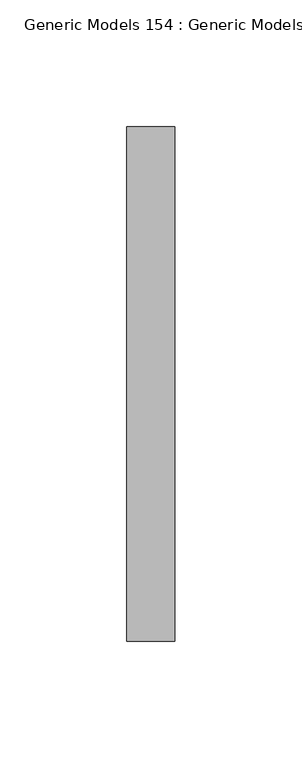
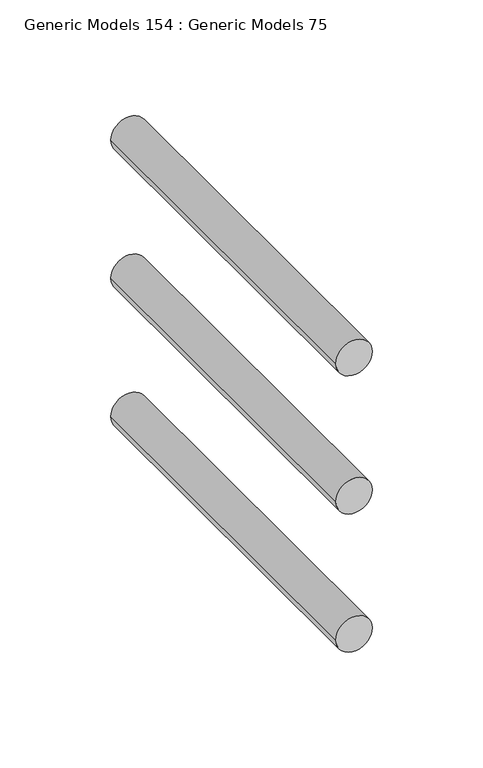
"""IFC4 building model written with IfcOpenShell, lengths in millimetres: proxy geometry, Generic Models 154 : Generic Models 75."""

from ifc_helpers import new_model, si_unit, point, frame, frame_2d, origin, place, context, project, spatial, circle_curve, trimmed, segment, composite_curve, outline, extrude, source, transform, mapped, element, save


def generic_models_154_generic_models_75_05dde245(model_context):
    return source(origin(), model_context, "Body", "SweptSolid", [
        extrude(outline(composite_curve([segment(trimmed(circle_curve(frame_2d((271689.5125, 31705.5346032)), 9.525), [point((271689.5125, 31715.0596032))], [point((271689.5125, 31696.0096032))], False, "CARTESIAN"), True, "CONTINUOUS"), segment(trimmed(circle_curve(frame_2d((271689.5125, 31705.5346032)), 9.525), [point((271689.5125, 31696.0096032))], [point((271689.5125, 31715.0596032))], False, "CARTESIAN"), True, "CONTINUOUS")], self_intersect=False)), frame((0.0, 36305.8207942, 0.0), z_axis=(0.0, 1.0, 0.0), x_axis=(0.0, 0.0, 1.0)), (0.0, 0.0, 1.0), 203.2),
        extrude(outline(composite_curve([segment(trimmed(circle_curve(frame_2d((271765.7125, 31705.5346032)), 9.525), [point((271765.7125, 31715.0596032))], [point((271765.7125, 31696.0096032))], False, "CARTESIAN"), True, "CONTINUOUS"), segment(trimmed(circle_curve(frame_2d((271765.7125, 31705.5346032)), 9.525), [point((271765.7125, 31696.0096032))], [point((271765.7125, 31715.0596032))], False, "CARTESIAN"), True, "CONTINUOUS")], self_intersect=False)), frame((0.0, 36305.8207942, 0.0), z_axis=(0.0, 1.0, 0.0), x_axis=(0.0, 0.0, 1.0)), (0.0, 0.0, 1.0), 203.2),
        extrude(outline(composite_curve([segment(trimmed(circle_curve(frame_2d((271841.9125, 31705.5346032)), 9.525), [point((271841.9125, 31715.0596032))], [point((271841.9125, 31696.0096032))], False, "CARTESIAN"), True, "CONTINUOUS"), segment(trimmed(circle_curve(frame_2d((271841.9125, 31705.5346032)), 9.525), [point((271841.9125, 31696.0096032))], [point((271841.9125, 31715.0596032))], False, "CARTESIAN"), True, "CONTINUOUS")], self_intersect=False)), frame((0.0, 36305.8207942, 0.0), z_axis=(0.0, 1.0, 0.0), x_axis=(0.0, 0.0, 1.0)), (0.0, 0.0, 1.0), 203.2),
    ])


if __name__ == "__main__":
    model = new_model("IFC4")
    model_context = context("Model", 3, world=origin())
    ifc_project = project(units=[si_unit("LENGTHUNIT", "METRE", prefix="MILLI")], contexts=[model_context])
    site = spatial("IfcSite", under=ifc_project)
    building = spatial("IfcBuilding", under=site)
    placement = place(None, origin())
    generic_models_154_generic_models_75_shape = generic_models_154_generic_models_75_05dde245(model_context)
    element("IfcBuildingElementProxy", 1, Name="Generic Models 154 : Generic Models 75", ObjectType="Generic Models 154 : Generic Models 75", at=placement, inside=building, context=model_context, shape_type="MappedRepresentation", body=[
        mapped(generic_models_154_generic_models_75_shape, transform((0.0, 0.0, 0.0), x_axis=(1.0, 0.0, 0.0), y_axis=(0.0, 1.0, 0.0), z_axis=(0.0, 0.0, 1.0))),
    ])
    save(model, "model.ifc")
